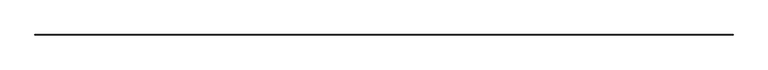
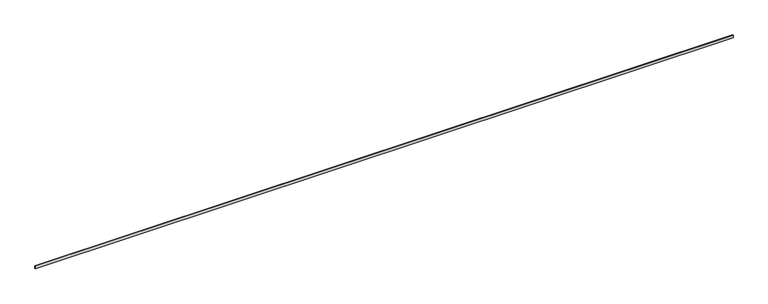
"""IFC4 building model written with IfcOpenShell, lengths in millimetres: proxy geometry, Generic Models 7:Generic Models 1:1:Generic Models 1:1 : Generic Models 7:Generic Models 1:337419:25 : Generic Models 7:Generic Models 1:1:Generic Models 1:1 : Generic Models 7:Generic Models 1:337419:306201."""

from ifc_helpers import new_model, si_unit, frame, origin, place, context, project, spatial, polyline, outline, extrude, source, transform, mapped, element, save


def generic_models_30f5fbb0(model_context):
    return source(origin(), model_context, "Body", "SweptSolid", [
        extrude(outline(polyline([(596062.696379, -578873.6913841), (596062.696379, -578886.3913841), (566081.674689, -578886.3913841), (566081.674689, -578873.6913841), (596062.696379, -578873.6913841)])), frame((0.0, 0.0, -158.1372439), z_axis=(0.0, 0.0, 1.0), x_axis=(1.0, 0.0, 0.0)), (0.0, 0.0, 1.0), 131.348355),
    ])


if __name__ == "__main__":
    model = new_model("IFC4")
    model_context = context("Model", 3, world=origin())
    ifc_project = project(units=[si_unit("LENGTHUNIT", "METRE", prefix="MILLI")], contexts=[model_context])
    site = spatial("IfcSite", under=ifc_project)
    building = spatial("IfcBuilding", under=site)
    placement = place(None, origin())
    generic_models_shape = generic_models_30f5fbb0(model_context)
    element("IfcBuildingElementProxy", 1, Name="Generic Models 7:Generic Models 1:1:Generic Models 1:1 : Generic Models 7:Generic Models 1:337419:25 : Generic Models 7:Generic Models 1:1:Generic Models 1:1 : Generic Models 7:Generic Models 1:337419:306201", ObjectType="Generic Models 7:Generic Models 1:1:Generic Models 1:1 : Generic Models 7:Generic Models 1:337419:25 : Generic Models 7:Generic Models 1:1:Generic Models 1:1 : Generic Models 7:Generic Models 1:337419:306201", at=placement, inside=building, context=model_context, shape_type="MappedRepresentation", body=[
        mapped(generic_models_shape, transform((0.0, 0.0, 0.0), x_axis=(1.0, 0.0, 0.0), y_axis=(0.0, 1.0, 0.0), z_axis=(0.0, 0.0, 1.0))),
    ])
    save(model, "model.ifc")

# Revit data of these elements
# Type "Generic Models 7:Generic Models 1:1:Generic Models 1:1 : Generic Models 7:Generic Models 1:337419:25 : Generic Models 7:Generic Models 1:1:Generic Models 1:1 : Generic Models 7:Generic Models 1:337419:306201"
#   NameOverride = "Generic Models 7:Generic Models 1:1:Generic Models 1:1 : Generic Models 7:Generic Models 1:337419:306201"
#   ObjectTypeOverride = "Generic Models 1:1 : Generic Models 7:Generic Models 1:337419"
#   Reference = "Generic Models 1"
#   Tag = "306201"
# Element 1 (IfcBuildingElementProxy, "Generic Models 7:Generic Models 1:1:Generic Models 1:1 : Generic Models 7:Generic Models 1:337419:25 : Generic Models 7:Generic Models 1:1:Generic Models 1:1 : Generic Models 7:Generic Models 1:337419:306201")
#   Materials on its faces: "COMPRESSIBLE JOINT FILLER"
# Materials
#   "COMPRESSIBLE JOINT FILLER": class "Generic", colour RGB 252 247 148, transparency 0, Cost = 0
